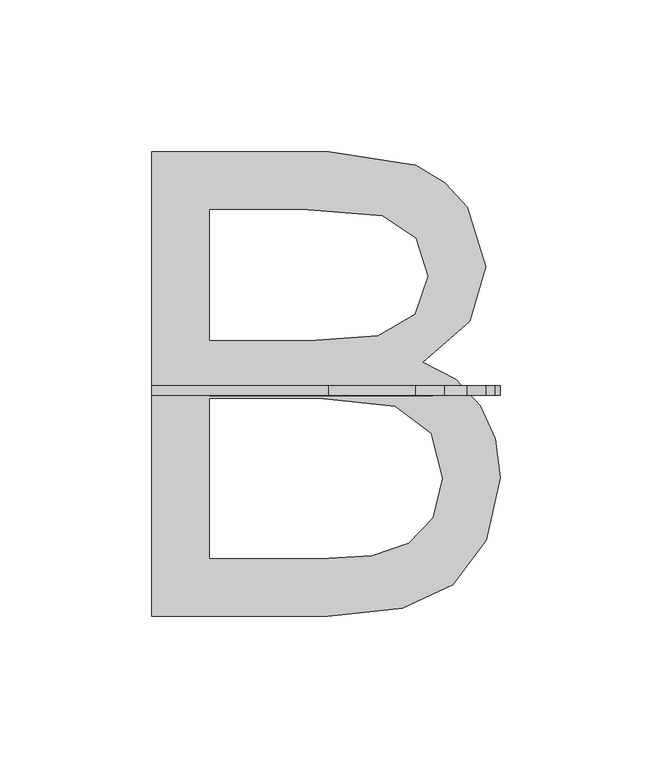
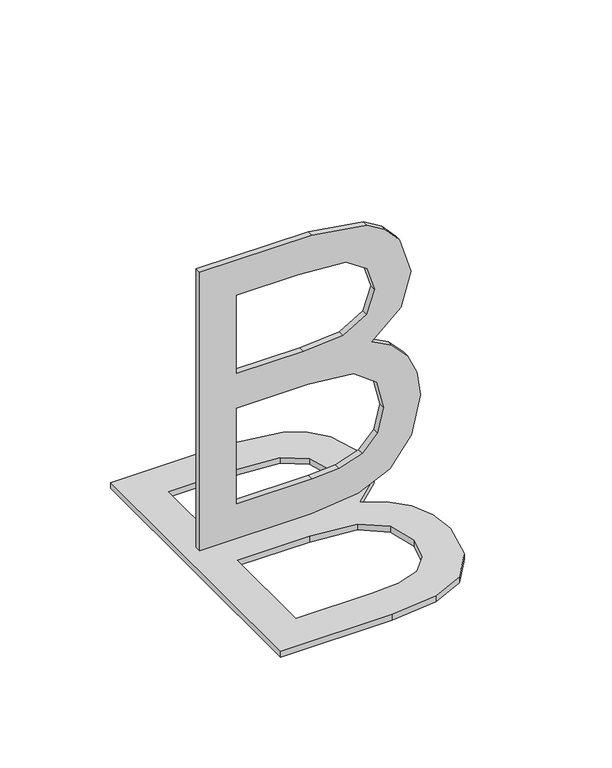
"""IFC4 building model written with IfcOpenShell, lengths in millimetres: proxy geometry, Grid Number1_FedEx : Grid Number1_FedEx."""

from ifc_helpers import new_model, si_unit, frame, origin, origin_with_axes, place, context, project, spatial, polyline, outline, extrude, source, transform, mapped, element, save


def entourage_4d3ed2b6(model_context):
    return source(origin(), model_context, "Body", "SweptSolid", [
        extrude(outline(polyline([(-161.8965342, 146.5840649), (-161.8965342, 299.6794816), (-103.476579, 299.6794816), (-74.8646304, 295.1755759), (-65.2494459, 289.461596), (-57.970312, 281.3274675), (-51.8592034, 261.7420187), (-56.9985149, 243.8572148), (-72.5285798, 230.3081209), (-61.6846325, 224.6455341), (-53.6719787, 216.0301792), (-48.7242234, 205.0320527), (-47.0749717, 192.2211508), (-51.5788773, 171.6452165), (-62.7358553, 156.9935067), (-79.3872245, 149.2191301), (-103.9251007, 146.5840649), (-161.8965342, 146.5840649)]), holes=[polyline([(-142.7596071, 237.4844686), (-107.8122891, 237.4844686), (-87.4045504, 239.1290482), (-75.1262681, 246.2119539), (-70.9961305, 258.6771202), (-74.845942, 271.160975), (-85.8721012, 278.5428951), (-110.4660426, 280.5425545), (-142.7596071, 280.5425545), (-142.7596071, 237.4844686)]), polyline([(-142.7596071, 165.720992), (-103.5139558, 165.720992), (-89.3107678, 166.4685282), (-77.2941231, 170.6360426), (-69.3328624, 179.1392671), (-66.2118987, 192.0342667), (-69.8748262, 206.9102374), (-81.7419636, 215.78723), (-105.3827964, 218.3475415), (-142.7596071, 218.3475415), (-142.7596071, 165.720992)])]), origin_with_axes(), (0.0, 0.0, 1.0), 3.175),
        extrude(outline(polyline([(14.4798932, -161.8965342), (14.4798932, -103.9251007), (17.1149584, -79.3872245), (24.889335, -62.7358553), (39.5410448, -51.5788773), (60.1169791, -47.0749717), (72.927881, -48.7242234), (83.9260075, -53.6719787), (92.5413624, -61.6846325), (98.2039492, -72.5285798), (111.7530431, -56.9985149), (129.637847, -51.8592034), (149.2232959, -57.970312), (157.3574243, -65.2494459), (163.0714042, -74.8646304), (167.5753099, -103.476579), (167.5753099, -161.8965342), (14.4798932, -161.8965342)]), holes=[polyline([(33.6168203, -142.7596071), (86.2433698, -142.7596071), (86.2433698, -105.3827964), (83.6830583, -81.7419636), (74.8060657, -69.8748262), (59.9300951, -66.2118987), (47.0350954, -69.3328624), (38.5318709, -77.2941231), (34.3643565, -89.3107678), (33.6168203, -103.5139558), (33.6168203, -142.7596071)]), polyline([(105.3802969, -142.7596071), (148.4383828, -142.7596071), (148.4383828, -110.4660426), (146.4387235, -85.8721012), (139.0568033, -74.845942), (126.5729486, -70.9961305), (114.1077822, -75.1262681), (107.0248766, -87.4045504), (105.3802969, -107.8122891), (105.3802969, -142.7596071)])]), frame((0.0, 219.3456765, 0.0), z_axis=(0.0, 1.0, 0.0), x_axis=(0.0, 0.0, 1.0)), (0.0, 0.0, 1.0), 3.175),
    ])


if __name__ == "__main__":
    model = new_model("IFC4")
    model_context = context("Model", 3, world=origin())
    ifc_project = project(units=[si_unit("LENGTHUNIT", "METRE", prefix="MILLI")], contexts=[model_context])
    site = spatial("IfcSite", under=ifc_project)
    building = spatial("IfcBuilding", under=site)
    placement = place(None, origin())
    entourage_shape = entourage_4d3ed2b6(model_context)
    element("IfcBuildingElementProxy", 1, Name="Grid Number1_FedEx : Grid Number1_FedEx", ObjectType="Grid Number1_FedEx : Grid Number1_FedEx", at=placement, inside=building, context=model_context, shape_type="MappedRepresentation", body=[
        mapped(entourage_shape, transform((0.0, 0.0, 0.0), x_axis=(1.0, 0.0, 0.0), y_axis=(0.0, 1.0, 0.0), z_axis=(0.0, 0.0, 1.0))),
    ])
    save(model, "model.ifc")

# Revit data of these elements
# Type "Grid Number1_FedEx : Grid Number1_FedEx"
#   Grid [instance default] = "S.8"
#   Label Width [instance default] = 1' - 0"
#   Half Box Width2 [instance default] = 0' - 6.13846"
#   Half Box Width [instance default] = 0' - 6"
#   Robust [instance default] = yes
#   Height = 0
#   Assembly Code = ""
# Element 1 (IfcBuildingElementProxy, "Grid Number1_FedEx : Grid Number1_FedEx")
#   Grid = "B"
#   Robust = no
#   Materials on its faces: "Letter"
# Materials
#   "Letter": class "Unassigned", colour RGB 178 187 30, transparency 0, Comments = "Rendering appearance not upgraded "
